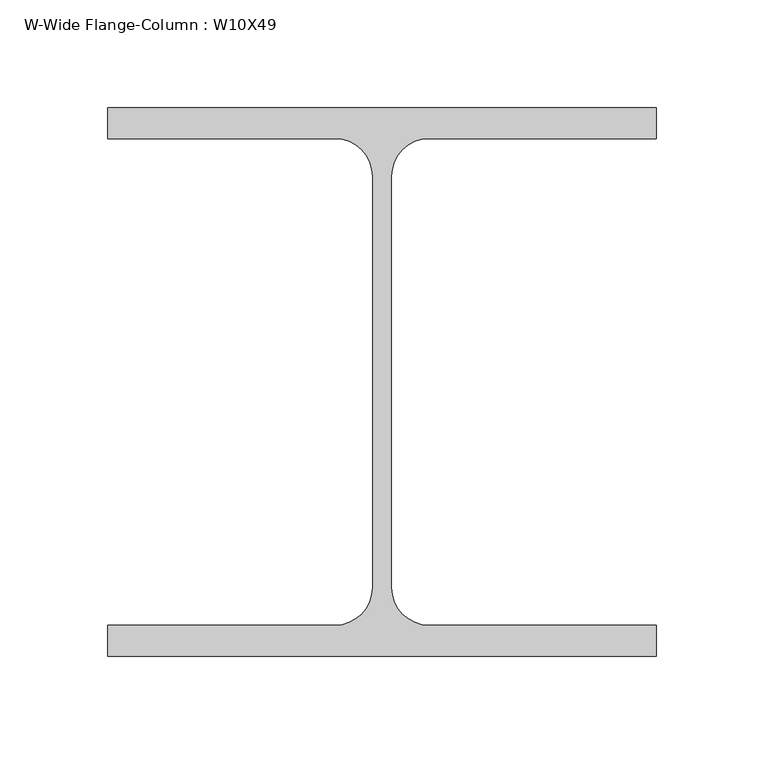
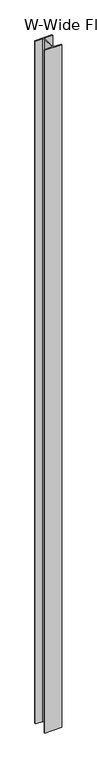
"""IFC4 building model written with IfcOpenShell, lengths in millimetres: column geometry, W-Wide Flange-Column : W10X49."""

from ifc_helpers import new_model, si_unit, point, frame, frame_2d, origin, place, context, project, spatial, polyline, circle_curve, trimmed, segment, composite_curve, outline, extrude, source, transform, mapped, element, save


def w_wide_flange_column_w10x49_cbcdba05(model_context):
    return source(origin(), model_context, "Body", "SweptSolid", [
        extrude(outline(composite_curve([segment(polyline([(127.0, 127.0), (127.0, 112.776), (21.844, 112.776)]), True, "CONTINUOUS"), segment(trimmed(circle_curve(frame_2d((21.844, 95.25)), 17.526), [point((21.844, 112.776))], [point((4.318, 95.25))], True, "CARTESIAN"), True, "CONTINUOUS"), segment(polyline([(4.318, 95.25), (4.318, -95.25)]), True, "CONTINUOUS"), segment(trimmed(circle_curve(frame_2d((21.844, -95.25)), 17.526), [point((4.318, -95.25))], [point((21.844, -112.776))], True, "CARTESIAN"), True, "CONTINUOUS"), segment(polyline([(21.844, -112.776), (127.0, -112.776), (127.0, -127.0), (-127.0, -127.0), (-127.0, -112.776), (-21.844, -112.776)]), True, "CONTINUOUS"), segment(trimmed(circle_curve(frame_2d((-21.844, -95.25)), 17.526), [point((-21.844, -112.776))], [point((-4.318, -95.25))], True, "CARTESIAN"), True, "CONTINUOUS"), segment(polyline([(-4.318, -95.25), (-4.318, 95.25)]), True, "CONTINUOUS"), segment(trimmed(circle_curve(frame_2d((-21.844, 95.25)), 17.526), [point((-4.318, 95.25))], [point((-21.844, 112.776))], True, "CARTESIAN"), True, "CONTINUOUS"), segment(polyline([(-21.844, 112.776), (-127.0, 112.776), (-127.0, 127.0), (127.0, 127.0)]), True, "CONTINUOUS")], self_intersect=False)), frame((0.0, 0.0, 12566.65), z_axis=(0.0, 0.0, 1.0), x_axis=(1.0, 0.0, 0.0)), (0.0, 0.0, 1.0), 10750.55),
    ])


if __name__ == "__main__":
    model = new_model("IFC4")
    model_context = context("Model", 3, world=origin())
    ifc_project = project(units=[si_unit("LENGTHUNIT", "METRE", prefix="MILLI")], contexts=[model_context])
    site = spatial("IfcSite", under=ifc_project)
    building = spatial("IfcBuilding", under=site)
    placement = place(None, origin())
    w_wide_flange_column_w10x49_shape = w_wide_flange_column_w10x49_cbcdba05(model_context)
    element("IfcColumn", 1, ObjectType="W-Wide Flange-Column : W10X49", at=placement, inside=building, context=model_context, shape_type="MappedRepresentation", body=[
        mapped(w_wide_flange_column_w10x49_shape, transform((0.0, 0.0, 0.0), x_axis=(1.0, 0.0, 0.0), y_axis=(0.0, 1.0, 0.0), z_axis=(0.0, 0.0, 1.0))),
    ])
    save(model, "model.ifc")

# Revit data of these elements
# Type "W-Wide Flange-Column : W10X49"
#   Assembly Code = "B10"
#   W = 49
#   bf = 0' - 10"
#   d = 0' - 10"
#   k = 0' - 1 1/4"
#   kr = 0' - 0.69"
#   tf = 0' - 0.56"
#   tw = 0' - 0.34"
#   A = 0.1 SF
#   Structural Material [instance default] = Steel ASTM A992
# Element 1 (IfcColumn, "W-Wide Flange-Column : W10X49")
#   Materials on its faces: "Steel ASTM A992"
# Materials
#   "Steel ASTM A992": class "Metal", colour RGB 199 199 199, transparency 0, Description = "Structural steel 50ksi", Cost = 0
